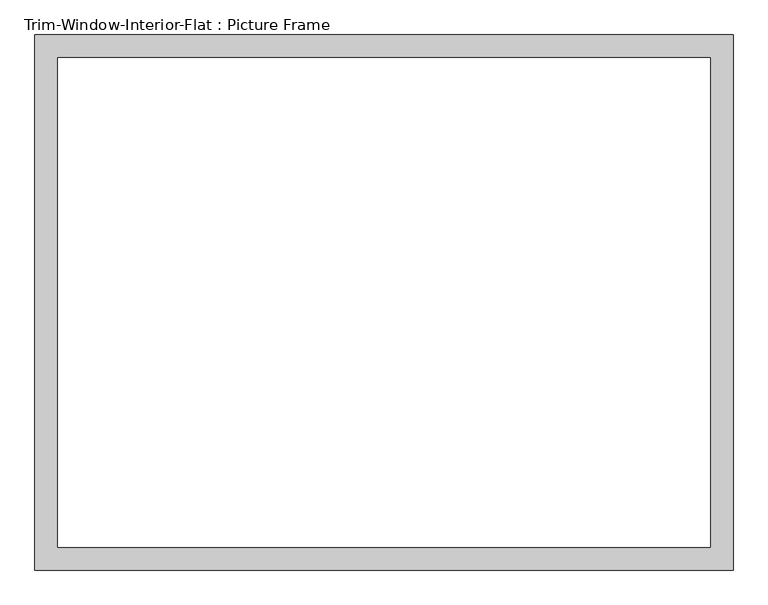
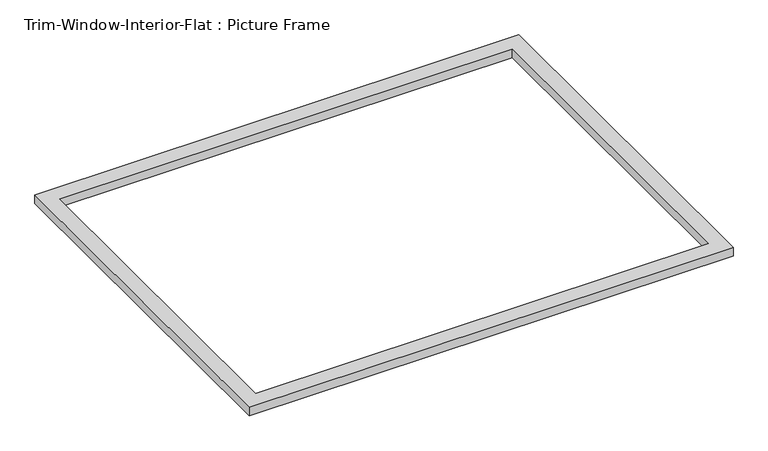
"""IFC4 building model written with IfcOpenShell, lengths in millimetres: proxy geometry, Trim-Window-Interior-Flat : Picture Frame."""

from ifc_helpers import new_model, si_unit, origin, origin_with_axes, place, context, project, spatial, polyline, outline, extrude, source, transform, mapped, element, save


def trim_window_interior_flat_picture_frame_4bb1ca52(model_context):
    return source(origin(), model_context, "Body", "SweptSolid", [
        extrude(outline(polyline([(869.95, 44.45), (869.95, -1289.05), (-869.95, -1289.05), (-869.95, 44.45), (869.95, 44.45)]), holes=[polyline([(812.8, -12.7), (-812.8, -12.7), (-812.8, -1231.9), (812.8, -1231.9), (812.8, -12.7)])]), origin_with_axes(), (0.0, 0.0, 1.0), 31.75),
    ])


if __name__ == "__main__":
    model = new_model("IFC4")
    model_context = context("Model", 3, world=origin())
    ifc_project = project(units=[si_unit("LENGTHUNIT", "METRE", prefix="MILLI")], contexts=[model_context])
    site = spatial("IfcSite", under=ifc_project)
    building = spatial("IfcBuilding", under=site)
    placement = place(None, origin())
    trim_window_interior_flat_picture_frame_shape = trim_window_interior_flat_picture_frame_4bb1ca52(model_context)
    element("IfcBuildingElementProxy", 1, Name="Trim-Window-Interior-Flat : Picture Frame", ObjectType="Trim-Window-Interior-Flat : Picture Frame", at=placement, inside=building, context=model_context, shape_type="MappedRepresentation", body=[
        mapped(trim_window_interior_flat_picture_frame_shape, transform((0.0, 0.0, 0.0), x_axis=(1.0, 0.0, 0.0), y_axis=(0.0, 1.0, 0.0), z_axis=(0.0, 0.0, 1.0))),
    ])
    save(model, "model.ifc")

# Revit data of these elements
# Type "Trim-Window-Interior-Flat : Picture Frame"
#   Trim Thickness_Picture Frame = 0' - 1 1/4"
#   Trim Width = 0' - 2 1/4"
#   Trim Thickness_with Sill = 0' - 0 3/4"
#   Sill Thickness = 0' - 1 1/4"
#   Opening Width [instance default] = 2' - 0"
#   Opening Height [instance default] = 3' - 0"
#   Default Elevation = 4' - 0"
#   Sill = no
#   Picture Frame = yes
#   Trim Material [instance default] = none
# Element 1 (IfcBuildingElementProxy, "Trim-Window-Interior-Flat : Picture Frame")
#   Opening Width = 5' - 5"
#   Opening Height = 4' - 1"
#   Trim Material = 1X WOOD COMPOSITE TRIM
#   Materials on its faces: "1X WOOD COMPOSITE TRIM"
# Materials
#   "1X WOOD COMPOSITE TRIM": class "Generic", colour RGB 88 61 61, transparency 0, Cost = 0
